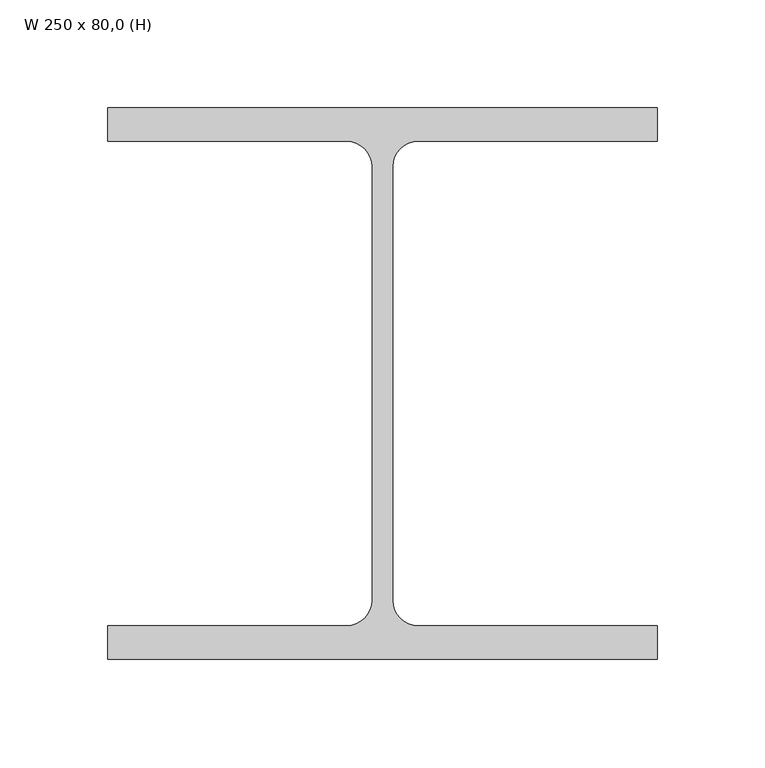
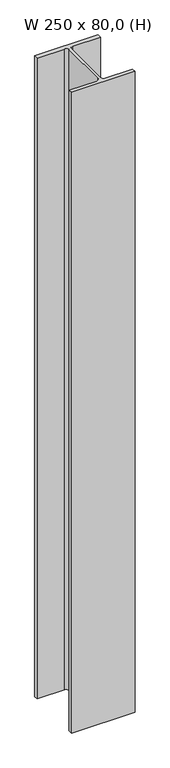
"""IFC4 building model written with IfcOpenShell, lengths in millimetres: column geometry, Pilar de Aço - H : W 250 x 80,0 (H)."""

from ifc_helpers import new_model, si_unit, point, frame_2d, origin, origin_with_axes, place, context, project, spatial, polyline, circle_curve, trimmed, segment, composite_curve, outline, extrude, source, transform, mapped, element, save


def w_250_x_80_0_h_aea14ab2(model_context):
    return source(origin(), model_context, "Body", "SweptSolid", [
        extrude(outline(composite_curve([segment(polyline([(127.5, 128.0), (127.5, 112.4), (16.6, 112.4)]), True, "CONTINUOUS"), segment(trimmed(circle_curve(frame_2d((16.6, 100.5)), 11.9), [point((16.6, 112.4))], [point((4.7, 100.5))], True, "CARTESIAN"), True, "CONTINUOUS"), segment(polyline([(4.7, 100.5), (4.7, -100.5)]), True, "CONTINUOUS"), segment(trimmed(circle_curve(frame_2d((16.6, -100.5)), 11.9), [point((4.7, -100.5))], [point((16.6, -112.4))], True, "CARTESIAN"), True, "CONTINUOUS"), segment(polyline([(16.6, -112.4), (127.5, -112.4), (127.5, -128.0), (-127.5, -128.0), (-127.5, -112.4), (-16.6, -112.4)]), True, "CONTINUOUS"), segment(trimmed(circle_curve(frame_2d((-16.6, -100.5)), 11.9), [point((-16.6, -112.4))], [point((-4.7, -100.5))], True, "CARTESIAN"), True, "CONTINUOUS"), segment(polyline([(-4.7, -100.5), (-4.7, 100.5)]), True, "CONTINUOUS"), segment(trimmed(circle_curve(frame_2d((-16.6, 100.5)), 11.9), [point((-4.7, 100.5))], [point((-16.6, 112.4))], True, "CARTESIAN"), True, "CONTINUOUS"), segment(polyline([(-16.6, 112.4), (-127.5, 112.4), (-127.5, 128.0), (127.5, 128.0)]), True, "CONTINUOUS")], self_intersect=False)), origin_with_axes(), (0.0, 0.0, 1.0), 2720.0),
    ])


if __name__ == "__main__":
    model = new_model("IFC4")
    model_context = context("Model", 3, world=origin())
    ifc_project = project(units=[si_unit("LENGTHUNIT", "METRE", prefix="MILLI")], contexts=[model_context])
    site = spatial("IfcSite", under=ifc_project)
    building = spatial("IfcBuilding", under=site)
    placement = place(None, origin())
    w_250_x_80_0_h_shape = w_250_x_80_0_h_aea14ab2(model_context)
    element("IfcColumn", 1, ObjectType="Pilar de Aço - H : W 250 x 80,0 (H)", at=placement, inside=building, context=model_context, shape_type="MappedRepresentation", body=[
        mapped(w_250_x_80_0_h_shape, transform((0.0, 0.0, 0.0), x_axis=(1.0, 0.0, 0.0), y_axis=(0.0, 1.0, 0.0), z_axis=(0.0, 0.0, 1.0))),
    ])
    save(model, "model.ifc")

# Revit data of these elements
# Type "Pilar de Aço - H : W 250 x 80,0 (H)"
#   SINAPI = ""
#   Área da seção = 101.9 m²
#   tw = 0.94 cm
#   tf = 1.56 cm
#   h = 22.48 cm
#   d' = 20.10 cm
#   d = 25.60 cm
#   bf = 25.50 cm
#   R = 1.19 cm
#   Massa Linear kg/m = 80
#   Aço = Metal - Aço 345MPa
#   Assembly Code = ""
# Materials
#   "Metal - Aço 345MPa": class "Metal", colour RGB 189 187 185, transparency 0, Cost = 0
